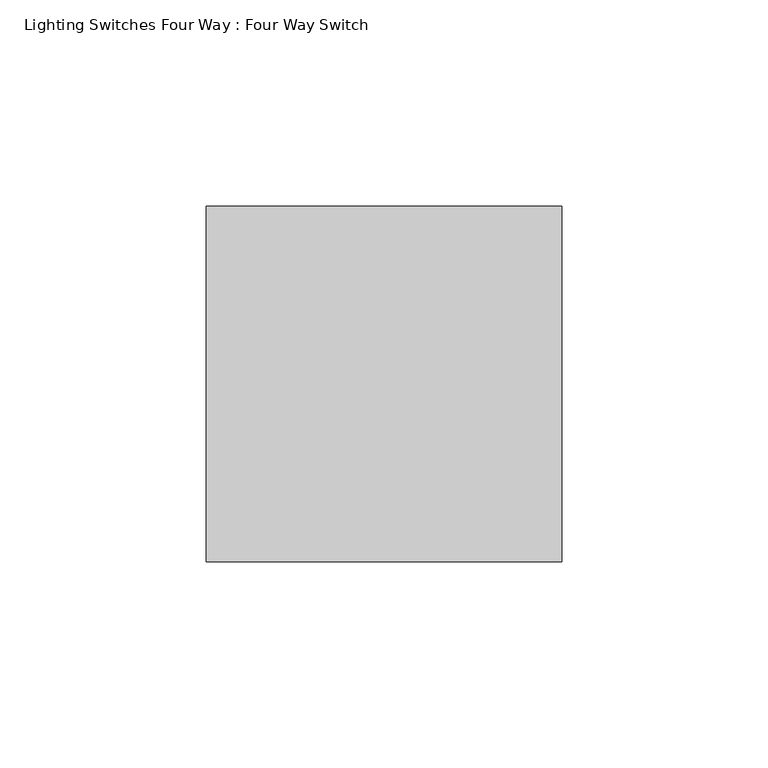
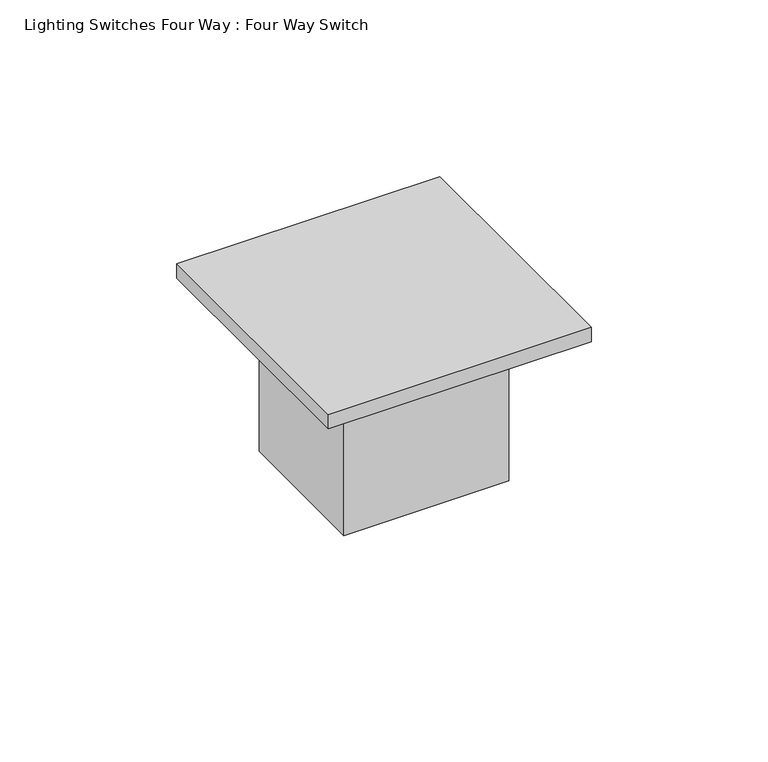
"""IFC4 building model written with IfcOpenShell, lengths in millimetres: switching device geometry, Lighting Switches Four Way : Four Way Switch."""

from ifc_helpers import new_model, si_unit, frame, origin, origin_with_axes, place, context, project, spatial, polyline, outline, extrude, source, transform, mapped, element, save


def lighting_switches_four_way_four_way_switch_ab144c04(model_context):
    return source(origin(), model_context, "Body", "SweptSolid", [
        extrude(outline(polyline([(43.0, -86.0), (-43.0, -86.0), (-43.0, 0.0), (43.0, 0.0), (43.0, -86.0)])), origin_with_axes(), (0.0, 0.0, 1.0), 5.0),
        extrude(outline(polyline([(27.0, -67.0), (-27.0, -67.0), (-27.0, -19.0), (27.0, -19.0), (27.0, -67.0)])), frame((0.0, 0.0, -54.0), z_axis=(0.0, 0.0, 1.0), x_axis=(1.0, 0.0, 0.0)), (0.0, 0.0, 1.0), 54.0),
    ])


if __name__ == "__main__":
    model = new_model("IFC4")
    model_context = context("Model", 3, world=origin())
    ifc_project = project(units=[si_unit("LENGTHUNIT", "METRE", prefix="MILLI")], contexts=[model_context])
    site = spatial("IfcSite", under=ifc_project)
    building = spatial("IfcBuilding", under=site)
    placement = place(None, origin())
    lighting_switches_four_way_four_way_switch_shape = lighting_switches_four_way_four_way_switch_ab144c04(model_context)
    element("IfcSwitchingDevice", 1, ObjectType="Lighting Switches Four Way : Four Way Switch", at=placement, inside=building, context=model_context, shape_type="MappedRepresentation", body=[
        mapped(lighting_switches_four_way_four_way_switch_shape, transform((0.0, 0.0, 0.0), x_axis=(1.0, 0.0, 0.0), y_axis=(0.0, 1.0, 0.0), z_axis=(0.0, 0.0, 1.0))),
    ])
    save(model, "model.ifc")

# Revit data of these elements
# Type "Lighting Switches Four Way : Four Way Switch"
#   Type Mark = "Lighting Switches Four Way"
#   Classification.OmniClass.21.Number = "21-04 50 40 10"
#   Classification.OmniClass.21.Description = "Lighting Control"
#   Classification.UniFormat.II.Description = "Lighting Control"
#   Classification.OmniClass.23.Number = "23-35 37 00"
#   Classification.OmniClass.23.Description = "Electrical Switches"
#   Classification.UniFormat.II.Number = "D5040.10"
#   COBie.Type.CreatedBy = "info@mma.ie"
#   COBie.Type.CreatedOn = "2017-07-25T10:15:16"
#   COBie.Type.Name = "Lighting Switches Four Way"
#   COBie.Type.Category = "23-35 37 00 : Electrical Switches"
#   COBie.Type.Description = "Lighting Switches Four Way_Four Way Switch"
#   COBie.Type.AssetType = "Fixed"
#   COBie.Type.Manufacturer = ""
#   COBie.Type.ModelNumber = ""
#   Label = "4"
#   Keynote = "26 36 13.D"
#   COBie.Type.ReplacementCost = 0
#   Switch Voltage [instance default] = 230 V
#   Default Elevation = 1200 mm
#   Apparent Load = 0 VA
#   4.W.S. Width = 86 mm
#   4.W.S. Height = 86 mm
#   4.W.S. Depth = 59 mm
#   COBie.Type = yes
#   Visibility 7 = no
#   Visibility 6 = no
#   Visibility 5 = no
#   Visibility 4 = yes
#   Visibility 3 = no
#   Visibility 2 = no
#   Visibility 1 = no
#   Ballast Number of Poles = 1
#   Load Classification = Other
#   4.W.S. Material = Metal - Chrome
# Materials
#   "Metal - Chrome": class "Metal", colour RGB 17 17 17, transparency 0, Comments = "Rendering appearance not upgraded "
